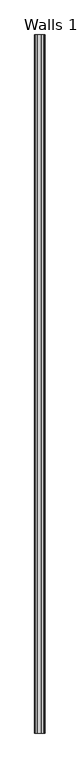
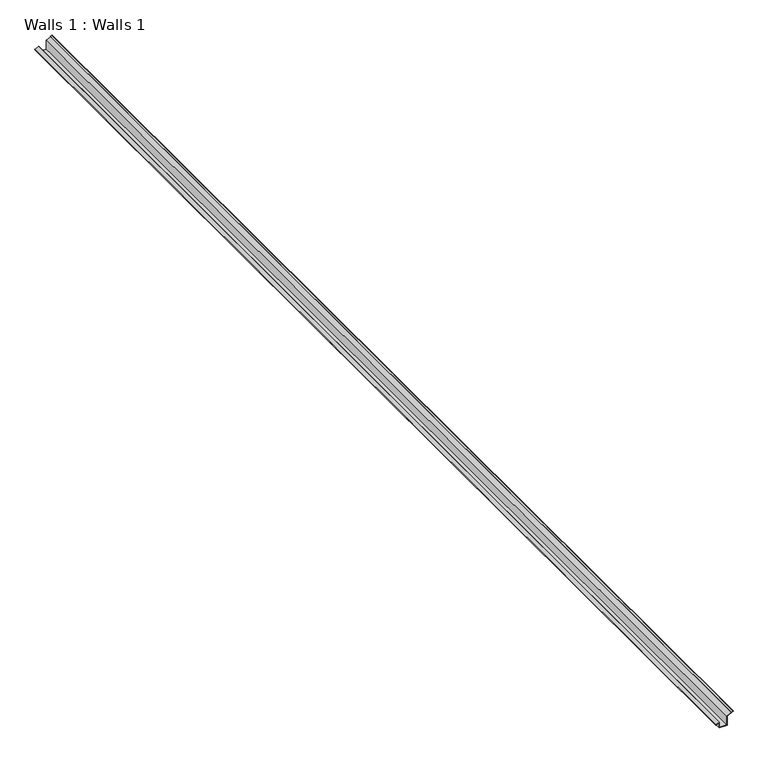
"""IFC4 building model written with IfcOpenShell, lengths in millimetres: proxy geometry, Walls 1 : Walls 1."""

from ifc_helpers import new_model, si_unit, point, frame, frame_2d, origin, place, context, project, spatial, polyline, circle_curve, trimmed, segment, composite_curve, outline, extrude, source, transform, mapped, element, save


def walls_1_walls_1_9406431e(model_context):
    return source(origin(), model_context, "Body", "SweptSolid", [
        extrude(outline(composite_curve([segment(polyline([(272183.225, 23413.2403278), (272258.5080898, 23413.2403278), (272234.8820297, 23365.9882076)]), True, "CONTINUOUS"), segment(trimmed(circle_curve(frame_2d((272231.5961214, 23367.6311618)), 3.6737572), [point((272234.8820297, 23365.9882076))], [point((272228.310213, 23369.2741159))], False, "CARTESIAN"), True, "CONTINUOUS"), segment(polyline([(272228.310213, 23369.2741159), (272235.1312142, 23382.9161183), (272236.5511174, 23382.2061667), (272229.7301162, 23368.5641643)]), True, "CONTINUOUS"), segment(trimmed(circle_curve(frame_2d((272231.5961214, 23367.6311618)), 2.0862572), [point((272229.7301162, 23368.5641643))], [point((272233.4621266, 23366.6981592))], True, "CARTESIAN"), True, "CONTINUOUS"), segment(polyline([(272233.4621266, 23366.6981592), (272255.9394609, 23411.6528278), (272181.6375, 23411.6528278), (272181.6375, 23513.2528278), (272305.7523861, 23513.2528278), (272344.022165, 23589.7923854)]), True, "CONTINUOUS"), segment(trimmed(circle_curve(frame_2d((272348.1219324, 23587.7425017)), 4.5836793), [point((272344.022165, 23589.7923854))], [point((272352.2216998, 23585.6926181))], False, "CARTESIAN"), True, "CONTINUOUS"), segment(polyline([(272352.2216998, 23585.6926181), (272342.3936698, 23566.0365581), (272340.9737666, 23566.7465097), (272350.8017966, 23586.4025696)]), True, "CONTINUOUS"), segment(trimmed(circle_curve(frame_2d((272348.1219324, 23587.7425017)), 2.9961793), [point((272350.8017966, 23586.4025696))], [point((272345.4420681, 23589.0824339))], True, "CARTESIAN"), True, "CONTINUOUS"), segment(polyline([(272345.4420681, 23589.0824339), (272306.7335151, 23511.6653278), (272183.225, 23511.6653278), (272183.225, 23413.2403278)]), True, "CONTINUOUS")], self_intersect=False)), frame((0.0, 25500.6656612, 0.0), z_axis=(0.0, 1.0, 0.0), x_axis=(0.0, 0.0, 1.0)), (0.0, 0.0, 1.0), 15480.9825),
    ])


if __name__ == "__main__":
    model = new_model("IFC4")
    model_context = context("Model", 3, world=origin())
    ifc_project = project(units=[si_unit("LENGTHUNIT", "METRE", prefix="MILLI")], contexts=[model_context])
    site = spatial("IfcSite", under=ifc_project)
    building = spatial("IfcBuilding", under=site)
    placement = place(None, origin())
    walls_1_walls_1_shape = walls_1_walls_1_9406431e(model_context)
    element("IfcBuildingElementProxy", 1, Name="Walls 1 : Walls 1", ObjectType="Walls 1 : Walls 1", at=placement, inside=building, context=model_context, shape_type="MappedRepresentation", body=[
        mapped(walls_1_walls_1_shape, transform((0.0, 0.0, 0.0), x_axis=(1.0, 0.0, 0.0), y_axis=(0.0, 1.0, 0.0), z_axis=(0.0, 0.0, 1.0))),
    ])
    save(model, "model.ifc")

# Revit data of these elements
# Element 1 (IfcBuildingElementProxy, "Walls 1 : Walls 1")
#   Materials on its faces: "SEAMLESS CONCEALED SHEET METAL GUTTER - (COLOR: GALVANIZED)"
# Materials
#   "SEAMLESS CONCEALED SHEET METAL GUTTER - (COLOR: GALVANIZED)": class "Generic", colour RGB 120 120 120, transparency 0, Cost = 0
